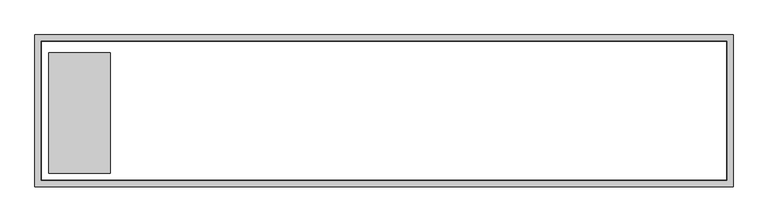
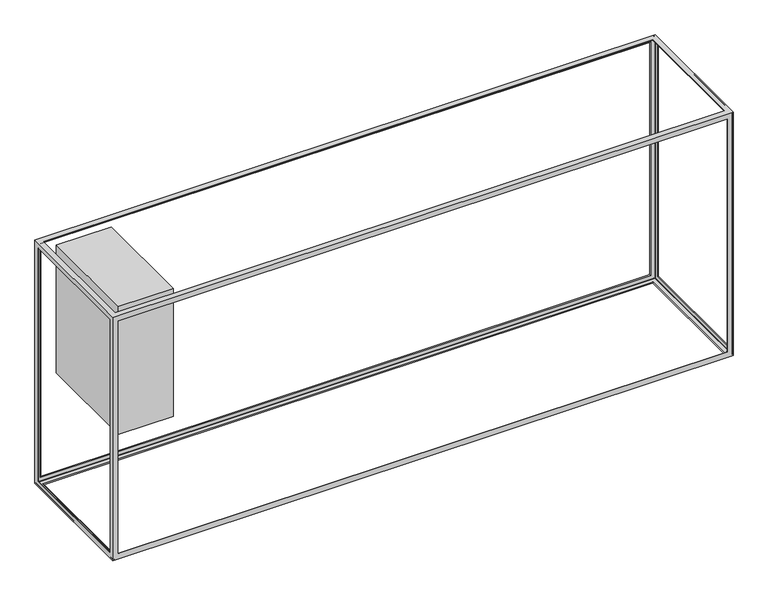
"""IFC4 building model written with IfcOpenShell, lengths in millimetres: beam geometry, Plumbing Bulkhead : EX. BULKHEAD 2."""

from ifc_helpers import new_model, si_unit, frame, origin, place, context, project, spatial, polyline, ellipse_curve, outline, extrude, source, transform, mapped, element, save
from ifc_brep_helpers import plane_surface, cylinder_surface, revolved_surface, advanced_brep


def beam_97812c56(model_context):
    return source(origin(), model_context, "Body", "SolidModel", [
        extrude(outline(polyline([(379.0365927, 673.1), (379.0365927, 66.5145898), (70.4236299, 66.5145898), (70.4236299, 673.1), (379.0365927, 673.1)])), frame((0.0, 0.0, 688.452765), z_axis=(0.0, 0.0, 1.0), x_axis=(1.0, 0.0, 0.0)), (0.0, 0.0, 1.0), 765.697235),
        advanced_brep(
        [(0.0, 0.0, 1454.15), (0.0, 762.0, 1454.15), (0.0, 762.0, 0.0), (0.0, 0.0, 0.0), (0.0, 31.75, 1422.4), (0.0, 31.75, 31.75), (0.0, 730.25, 31.75), (0.0, 730.25, 1422.4), (3505.2, 762.0, 1454.15), (3505.2, 762.0, 0.0), (3473.45, 762.0, 31.75), (3473.45, 762.0, 1422.4), (31.75, 762.0, 1422.4), (31.75, 762.0, 31.75), (3505.2, 0.0, 0.0), (3473.45, 730.25, 0.0), (31.75, 730.25, 0.0), (31.75, 31.75, 0.0), (3473.45, 31.75, 0.0), (3505.2, 0.0, 1454.15), (3473.45, 0.0, 1422.4), (3473.45, 0.0, 31.75), (31.75, 0.0, 31.75), (31.75, 0.0, 1422.4), (3.175, 28.575, 1425.575), (3.175, 28.575, 28.575), (3.175, 733.425, 28.575), (3.175, 733.425, 1425.575), (3505.2, 730.25, 31.75), (3502.025, 733.425, 28.575), (3502.025, 28.575, 28.575), (3505.2, 31.75, 31.75), (3505.2, 31.75, 1422.4), (3505.2, 730.25, 1422.4), (3502.025, 28.575, 1425.575), (3502.025, 733.425, 1425.575), (3476.625, 733.425, 3.175), (28.575, 733.425, 3.175), (28.575, 28.575, 3.175), (3476.625, 28.575, 3.175), (3500.4375, 4.7625, 3.175), (3500.4375, 757.2375, 3.175), (4.7625, 757.2375, 3.175), (4.7625, 4.7625, 3.175), (3501.560032, 758.360032, 3.639968), (3501.560032, 3.639968, 3.639968), (3502.025, 4.7625, 4.7625), (3502.025, 757.2375, 4.7625), (3500.4375, 758.825, 4.7625), (4.7625, 758.825, 4.7625), (3.639968, 758.360032, 3.639968), (3.175, 757.2375, 4.7625), (3.175, 4.7625, 4.7625), (3.639968, 3.639968, 3.639968), (4.7625, 3.175, 4.7625), (3500.4375, 3.175, 4.7625), (3500.4375, 758.825, 1449.3875), (4.7625, 758.825, 1449.3875), (3476.625, 758.825, 1425.575), (3476.625, 758.825, 28.575), (28.575, 758.825, 28.575), (28.575, 758.825, 1425.575), (3.639968, 758.360032, 1450.510032), (3.175, 757.2375, 1449.3875), (3502.025, 757.2375, 1449.3875), (3501.560032, 758.360032, 1450.510032), (3502.025, 4.7625, 1449.3875), (3500.4375, 3.175, 1449.3875), (3501.560032, 3.639968, 1450.510032), (3.175, 4.7625, 1449.3875), (4.7625, 3.175, 1449.3875), (3.639968, 3.639968, 1450.510032), (3476.625, 3.175, 1425.575), (3476.625, 3.175, 28.575), (28.575, 3.175, 28.575), (28.575, 3.175, 1425.575), (31.75, 31.75, 1454.15), (31.75, 730.25, 1454.15), (3473.45, 730.25, 1454.15), (3473.45, 31.75, 1454.15), (28.575, 733.425, 1450.975), (3476.625, 733.425, 1450.975), (4.7625, 4.7625, 1450.975), (4.7625, 757.2375, 1450.975), (3500.4375, 757.2375, 1450.975), (3500.4375, 4.7625, 1450.975), (28.575, 28.575, 1450.975), (3476.625, 28.575, 1450.975)],
        [
            (0, 1),
            (1, 2),
            (2, 3),
            (3, 0),
            (4, 5),
            (5, 6),
            (6, 7),
            (7, 4),
            (8, 9),
            (9, 2),
            (1, 8),
            (10, 11),
            (11, 12),
            (12, 13),
            (13, 10),
            (9, 14),
            (14, 3),
            (15, 16),
            (16, 17),
            (17, 18),
            (18, 15),
            (14, 19),
            (19, 0),
            (20, 21),
            (21, 22),
            (22, 23),
            (23, 20),
            (4, 24, ellipse_curve(frame((0.0, 28.575, 1425.575), z_axis=(0.0, -0.7071067811865464, -0.7071067811865487), x_axis=(0.0, 0.7071067811865487, -0.7071067811865464)), 4.4901281, 3.175)),
            (24, 25),
            (25, 5, ellipse_curve(frame((0.0, 28.575, 28.575), z_axis=(0.0, -0.7071067811865499, 0.7071067811865451), x_axis=(0.0, -0.7071067811865451, -0.7071067811865498)), 4.4901281, 3.175)),
            (25, 26),
            (26, 6, ellipse_curve(frame((0.0, 733.425, 28.575), z_axis=(0.0, -0.707106781186545, -0.70710678118655), x_axis=(0.0, -0.7071067811865501, 0.7071067811865449)), 4.4901281, 3.175)),
            (27, 7, ellipse_curve(frame((0.0, 733.425, 1425.575), z_axis=(0.0, 0.7071067811865487, -0.7071067811865464), x_axis=(0.0, -0.7071067811865465, -0.7071067811865487)), 4.4901281, 3.175)),
            (26, 27),
            (28, 29, ellipse_curve(frame((3505.2, 733.425, 28.575), z_axis=(0.0, -0.7071067811865429, -0.7071067811865522), x_axis=(0.0, -0.7071067811865521, 0.707106781186543)), 4.4901281, 3.175)),
            (29, 30),
            (30, 31, ellipse_curve(frame((3505.2, 28.575, 28.575), z_axis=(0.0, 0.7071067811865499, -0.7071067811865451), x_axis=(0.0, -0.7071067811865451, -0.70710678118655)), 4.4901281, 3.175)),
            (31, 28),
            (8, 19),
            (31, 32),
            (32, 33),
            (33, 28),
            (30, 34),
            (34, 32, ellipse_curve(frame((3505.2, 28.575, 1425.575), z_axis=(0.0, -0.7071067811865464, -0.7071067811865487), x_axis=(0.0, 0.7071067811865487, -0.7071067811865464)), 4.4901281, 3.175)),
            (33, 35, ellipse_curve(frame((3505.2, 733.425, 1425.575), z_axis=(0.0, 0.707106781186551, -0.7071067811865441), x_axis=(0.0, -0.7071067811865441, -0.7071067811865509)), 4.4901281, 3.175)),
            (35, 29),
            (15, 36, ellipse_curve(frame((3476.625, 733.425, 0.0), z_axis=(-0.7071067811865475, 0.7071067811865475, 0.0), x_axis=(-0.7071067811865476, -0.7071067811865474, 0.0)), 4.4901281, 3.175)),
            (36, 37),
            (37, 16, ellipse_curve(frame((28.575, 733.425, 0.0), z_axis=(0.7071067811865454, 0.7071067811865498, 0.0), x_axis=(-0.7071067811865497, 0.7071067811865454, 0.0)), 4.4901281, 3.175)),
            (37, 38),
            (38, 17, ellipse_curve(frame((28.575, 28.575, 0.0), z_axis=(-0.7071067811865498, 0.7071067811865452, 0.0), x_axis=(-0.7071067811865451, -0.7071067811865498, 0.0)), 4.4901281, 3.175)),
            (39, 18, ellipse_curve(frame((3476.625, 28.575, 0.0), z_axis=(-0.7071067811865475, -0.7071067811865475, 0.0), x_axis=(-0.7071067811865476, 0.7071067811865474, 0.0)), 4.4901281, 3.175)),
            (38, 39),
            (39, 36),
            (40, 41),
            (41, 42),
            (42, 43),
            (43, 40),
            (44, 41, ellipse_curve(frame((3500.4375, 757.2375, 4.7625), z_axis=(-0.7071067811865475, 0.7071067811865475, 0.0), x_axis=(0.7071067811865474, 0.7071067811865476, 0.0)), 2.245064, 1.5875)),
            (40, 45, ellipse_curve(frame((3500.4375, 4.7625, 4.7625), z_axis=(-0.7071067811865475, -0.7071067811865475, 0.0), x_axis=(-0.7071067811865474, 0.7071067811865476, 0.0)), 2.245064, 1.5875)),
            (45, 46, ellipse_curve(frame((3500.4375, 4.7625, 4.7625), z_axis=(0.0, -0.7071067811865499, 0.7071067811865451), x_axis=(0.0, 0.7071067811865451, 0.70710678118655)), 2.245064, 1.5875)),
            (46, 47),
            (47, 44, ellipse_curve(frame((3500.4375, 757.2375, 4.7625), z_axis=(0.0, 0.7071067811865429, 0.7071067811865522), x_axis=(0.0, 0.7071067811865521, -0.707106781186543)), 2.245064, 1.5875)),
            (48, 49),
            (49, 50, ellipse_curve(frame((4.7625, 757.2375, 4.7625), z_axis=(-0.7071067811865439, 0.0, 0.7071067811865511), x_axis=(0.7071067811865511, 0.0, 0.7071067811865438)), 2.245064, 1.5875)),
            (50, 42, ellipse_curve(frame((4.7625, 757.2375, 4.7625), z_axis=(-0.7071067811865454, -0.7071067811865498, 0.0), x_axis=(0.7071067811865497, -0.7071067811865454, 0.0)), 2.245064, 1.5875)),
            (44, 48, ellipse_curve(frame((3500.4375, 757.2375, 4.7625), z_axis=(0.7071067811865475, 0.0, 0.7071067811865476), x_axis=(0.7071067811865475, 0.0, -0.7071067811865475)), 2.245064, 1.5875)),
            (51, 52),
            (52, 53, ellipse_curve(frame((4.7625, 4.7625, 4.7625), z_axis=(0.0, -0.7071067811865499, 0.7071067811865451), x_axis=(0.0, 0.7071067811865451, 0.70710678118655)), 2.245064, 1.5875)),
            (53, 43, ellipse_curve(frame((4.7625, 4.7625, 4.7625), z_axis=(0.7071067811865498, -0.7071067811865452, 0.0), x_axis=(0.7071067811865451, 0.7071067811865498, 0.0)), 2.245064, 1.5875)),
            (50, 51, ellipse_curve(frame((4.7625, 757.2375, 4.7625), z_axis=(0.0, 0.707106781186545, 0.70710678118655), x_axis=(0.0, 0.7071067811865501, -0.7071067811865449)), 2.245064, 1.5875)),
            (53, 54, ellipse_curve(frame((4.7625, 4.7625, 4.7625), z_axis=(-0.7071067811865439, 0.0, 0.7071067811865511), x_axis=(0.7071067811865511, 0.0, 0.7071067811865438)), 2.245064, 1.5875)),
            (54, 55),
            (55, 45, ellipse_curve(frame((3500.4375, 4.7625, 4.7625), z_axis=(0.7071067811865475, 0.0, 0.7071067811865476), x_axis=(0.7071067811865475, 0.0, -0.7071067811865475)), 2.245064, 1.5875)),
            (48, 56),
            (56, 57),
            (57, 49),
            (58, 59),
            (59, 60),
            (60, 61),
            (61, 58),
            (57, 62, ellipse_curve(frame((4.7625, 757.2375, 1449.3875), z_axis=(0.7071067811865511, 0.0, 0.7071067811865439), x_axis=(-0.7071067811865438, 0.0, 0.7071067811865511)), 2.245064, 1.5875)),
            (62, 63, ellipse_curve(frame((4.7625, 757.2375, 1449.3875), z_axis=(0.0, -0.7071067811865487, 0.7071067811865464), x_axis=(0.0, 0.7071067811865465, 0.7071067811865487)), 2.245064, 1.5875)),
            (63, 51),
            (47, 64),
            (64, 65, ellipse_curve(frame((3500.4375, 757.2375, 1449.3875), z_axis=(0.0, -0.707106781186551, 0.7071067811865441), x_axis=(0.0, 0.7071067811865441, 0.7071067811865509)), 2.245064, 1.5875)),
            (65, 56, ellipse_curve(frame((3500.4375, 757.2375, 1449.3875), z_axis=(-0.7071067811865475, 0.0, 0.7071067811865475), x_axis=(0.7071067811865474, 0.0, 0.7071067811865476)), 2.245064, 1.5875)),
            (10, 59, ellipse_curve(frame((3476.625, 762.0, 28.575), z_axis=(0.7071067811865475, 0.0, 0.7071067811865476), x_axis=(0.7071067811865476, 0.0, -0.7071067811865475)), 4.4901281, 3.175)),
            (58, 11, ellipse_curve(frame((3476.625, 762.0, 1425.575), z_axis=(0.7071067811865475, 0.0, -0.7071067811865475), x_axis=(-0.7071067811865474, 0.0, -0.7071067811865476)), 4.4901281, 3.175)),
            (13, 60, ellipse_curve(frame((28.575, 762.0, 28.575), z_axis=(0.7071067811865439, 0.0, -0.7071067811865511), x_axis=(-0.7071067811865511, 0.0, -0.7071067811865438)), 4.4901281, 3.175)),
            (12, 61, ellipse_curve(frame((28.575, 762.0, 1425.575), z_axis=(-0.7071067811865511, 0.0, -0.7071067811865439), x_axis=(0.7071067811865438, 0.0, -0.7071067811865511)), 4.4901281, 3.175)),
            (46, 66),
            (66, 64),
            (35, 34),
            (55, 67),
            (67, 68, ellipse_curve(frame((3500.4375, 4.7625, 1449.3875), z_axis=(-0.7071067811865475, 0.0, 0.7071067811865475), x_axis=(0.7071067811865474, 0.0, 0.7071067811865476)), 2.245064, 1.5875)),
            (68, 66, ellipse_curve(frame((3500.4375, 4.7625, 1449.3875), z_axis=(0.0, 0.7071067811865464, 0.7071067811865487), x_axis=(0.0, -0.7071067811865487, 0.7071067811865464)), 2.245064, 1.5875)),
            (63, 69),
            (69, 52),
            (24, 27),
            (70, 54),
            (69, 71, ellipse_curve(frame((4.7625, 4.7625, 1449.3875), z_axis=(0.0, 0.7071067811865464, 0.7071067811865487), x_axis=(0.0, -0.7071067811865487, 0.7071067811865464)), 2.245064, 1.5875)),
            (71, 70, ellipse_curve(frame((4.7625, 4.7625, 1449.3875), z_axis=(0.7071067811865511, 0.0, 0.7071067811865439), x_axis=(-0.7071067811865438, 0.0, 0.7071067811865511)), 2.245064, 1.5875)),
            (72, 73),
            (73, 21, ellipse_curve(frame((3476.625, 0.0, 28.575), z_axis=(0.7071067811865475, 0.0, 0.7071067811865476), x_axis=(0.7071067811865476, 0.0, -0.7071067811865475)), 4.4901281, 3.175)),
            (20, 72, ellipse_curve(frame((3476.625, 0.0, 1425.575), z_axis=(0.7071067811865475, 0.0, -0.7071067811865475), x_axis=(-0.7071067811865474, 0.0, -0.7071067811865476)), 4.4901281, 3.175)),
            (73, 74),
            (74, 22, ellipse_curve(frame((28.575, 0.0, 28.575), z_axis=(0.7071067811865439, 0.0, -0.7071067811865511), x_axis=(-0.7071067811865511, 0.0, -0.7071067811865438)), 4.4901281, 3.175)),
            (74, 75),
            (75, 23, ellipse_curve(frame((28.575, 0.0, 1425.575), z_axis=(-0.7071067811865511, 0.0, -0.7071067811865439), x_axis=(0.7071067811865438, 0.0, -0.7071067811865511)), 4.4901281, 3.175)),
            (70, 67),
            (72, 75),
            (76, 77),
            (77, 78),
            (78, 79),
            (79, 76),
            (77, 80, ellipse_curve(frame((28.575, 733.425, 1454.15), z_axis=(0.707106781186548, 0.7071067811865469, 0.0), x_axis=(-0.707106781186547, 0.7071067811865478, 0.0)), 4.4901281, 3.175)),
            (80, 81),
            (81, 78, ellipse_curve(frame((3476.625, 733.425, 1454.15), z_axis=(-0.7071067811865469, 0.707106781186548, 0.0), x_axis=(-0.7071067811865481, -0.7071067811865468, 0.0)), 4.4901281, 3.175)),
            (82, 83),
            (83, 84),
            (84, 85),
            (85, 82),
            (80, 86),
            (86, 87),
            (87, 81),
            (65, 84, ellipse_curve(frame((3500.4375, 757.2375, 1449.3875), z_axis=(0.7071067811865469, -0.707106781186548, 0.0), x_axis=(0.7071067811865481, 0.7071067811865468, 0.0)), 2.245064, 1.5875)),
            (83, 62, ellipse_curve(frame((4.7625, 757.2375, 1449.3875), z_axis=(-0.707106781186548, -0.7071067811865469, 0.0), x_axis=(0.707106781186547, -0.7071067811865478, 0.0)), 2.245064, 1.5875)),
            (86, 76, ellipse_curve(frame((28.575, 28.575, 1454.15), z_axis=(0.7071067811865469, -0.707106781186548, 0.0), x_axis=(-0.7071067811865481, -0.7071067811865468, 0.0)), 4.4901281, 3.175)),
            (79, 87, ellipse_curve(frame((3476.625, 28.575, 1454.15), z_axis=(-0.707106781186548, -0.7071067811865469, 0.0), x_axis=(-0.707106781186547, 0.7071067811865478, 0.0)), 4.4901281, 3.175)),
            (71, 82, ellipse_curve(frame((4.7625, 4.7625, 1449.3875), z_axis=(-0.7071067811865469, 0.707106781186548, 0.0), x_axis=(0.7071067811865481, 0.7071067811865468, 0.0)), 2.245064, 1.5875)),
            (85, 68, ellipse_curve(frame((3500.4375, 4.7625, 1449.3875), z_axis=(0.707106781186548, 0.7071067811865469, 0.0), x_axis=(0.707106781186547, -0.7071067811865478, 0.0)), 2.245064, 1.5875)),
        ],
        [
            plane_surface(frame((0.0, 762.0, 0.0), z_axis=(-1.0, 0.0, 0.0), x_axis=(0.0, 0.0, 1.0))),
            plane_surface(frame((0.0, 762.0, 31.75), z_axis=(0.0, 1.0, 0.0), x_axis=(1.0, 0.0, 0.0))),
            plane_surface(frame((0.0, 762.0, 0.0), z_axis=(0.0, 0.0, -1.0), x_axis=(1.0, 0.0, 0.0))),
            plane_surface(frame((3505.2, 0.0, 0.0), z_axis=(0.0, -1.0, 0.0), x_axis=(0.0, 0.0, 1.0))),
            cylinder_surface(frame((0.0, 28.575, 0.0), z_axis=(0.0, 0.0, -1.0), x_axis=(0.0, 1.0, 0.0)), 3.175),
            cylinder_surface(frame((0.0, 0.0, 28.575), z_axis=(0.0, -1.0, 0.0), x_axis=(1.0, 0.0, 0.0)), 3.175),
            cylinder_surface(frame((0.0, 733.425, 0.0), z_axis=(0.0, 0.0, -1.0), x_axis=(0.0, -1.0, 0.0)), 3.175),
            cylinder_surface(frame((3505.2, 0.0, 28.575), z_axis=(0.0, -1.0, 0.0), x_axis=(-1.0, 0.0, 0.0)), 3.175),
            plane_surface(frame((3505.2, 762.0, 0.0), z_axis=(1.0, 0.0, 0.0), x_axis=(0.0, 0.0, 1.0))),
            cylinder_surface(frame((3505.2, 28.575, 0.0), z_axis=(0.0, 0.0, -1.0), x_axis=(0.0, 1.0, 0.0)), 3.175),
            cylinder_surface(frame((3505.2, 733.425, 0.0), z_axis=(0.0, 0.0, -1.0), x_axis=(0.0, -1.0, 0.0)), 3.175),
            cylinder_surface(frame((0.0, 733.425, 0.0), z_axis=(-1.0, 0.0, 0.0), x_axis=(0.0, -1.0, 0.0)), 3.175),
            cylinder_surface(frame((28.575, 0.0, 0.0), z_axis=(0.0, -1.0, 0.0), x_axis=(1.0, 0.0, 0.0)), 3.175),
            cylinder_surface(frame((0.0, 28.575, 0.0), z_axis=(-1.0, 0.0, 0.0), x_axis=(0.0, 1.0, 0.0)), 3.175),
            cylinder_surface(frame((3476.625, 0.0, 0.0), z_axis=(0.0, -1.0, 0.0), x_axis=(-1.0, 0.0, 0.0)), 3.175),
            plane_surface(frame((0.0, 733.425, 3.175), z_axis=(0.0, 0.0, 1.0), x_axis=(1.0, 0.0, 0.0))),
            revolved_surface(polyline([(3498.85, 758.8249999785978, 4.7625), (3498.85, 3.1750000214022047, 4.7625)]), (3500.4375, 0.0, 4.7625), (0.0, 1.0, 0.0)),
            revolved_surface(polyline([(3502.024999978598, 755.65, 4.7625), (3.175000021402197, 755.65, 4.7625)]), (0.0, 757.2375, 4.7625), (1.0, 0.0, 0.0)),
            revolved_surface(polyline([(6.35, 758.8249999785977, 4.7625), (6.35, 3.1750000214022, 4.7625)]), (4.7625, 0.0, 4.7625), (0.0, 1.0, 0.0)),
            revolved_surface(polyline([(3502.024999978598, 6.35, 4.7625), (3.175000021402197, 6.35, 4.7625)]), (0.0, 4.7625, 4.7625), (1.0, 0.0, 0.0)),
            plane_surface(frame((0.0, 758.825, 4.7625), z_axis=(0.0, -1.0, 0.0), x_axis=(1.0, 0.0, 0.0))),
            revolved_surface(polyline([(4.7625, 755.65, 1450.974999978598), (4.7625, 755.65, 3.1750000214022105)]), (4.7625, 757.2375, 0.0), (0.0, 0.0, 1.0)),
            revolved_surface(polyline([(3500.4375, 755.65, 1450.974999978598), (3500.4375, 755.65, 3.175000021402205)]), (3500.4375, 757.2375, 0.0), (0.0, 0.0, 1.0)),
            cylinder_surface(frame((3476.625, 762.0, 0.0), z_axis=(0.0, 0.0, -1.0), x_axis=(0.0, -1.0, 0.0)), 3.175),
            cylinder_surface(frame((0.0, 762.0, 28.575), z_axis=(-1.0, 0.0, 0.0), x_axis=(0.0, -1.0, 0.0)), 3.175),
            cylinder_surface(frame((28.575, 762.0, 0.0), z_axis=(0.0, 0.0, -1.0), x_axis=(0.0, -1.0, 0.0)), 3.175),
            plane_surface(frame((3502.025, 733.425, 0.0), z_axis=(-1.0, 0.0, 0.0), x_axis=(0.0, 0.0, 1.0))),
            revolved_surface(polyline([(3500.4375, 6.35, 1450.974999978598), (3500.4375, 6.35, 3.1750000214021994)]), (3500.4375, 4.7625, 0.0), (0.0, 0.0, 1.0)),
            plane_surface(frame((3.175, 757.2375, 0.0), z_axis=(1.0, 0.0, 0.0), x_axis=(0.0, 0.0, 1.0))),
            revolved_surface(polyline([(4.7625, 6.35, 1450.974999978598), (4.7625, 6.35, 3.1750000214021994)]), (4.7625, 4.7625, 0.0), (0.0, 0.0, 1.0)),
            cylinder_surface(frame((3476.625, 0.0, 0.0), z_axis=(0.0, 0.0, -1.0), x_axis=(0.0, 1.0, 0.0)), 3.175),
            cylinder_surface(frame((0.0, 0.0, 28.575), z_axis=(-1.0, 0.0, 0.0), x_axis=(0.0, 1.0, 0.0)), 3.175),
            cylinder_surface(frame((28.575, 0.0, 0.0), z_axis=(0.0, 0.0, -1.0), x_axis=(0.0, 1.0, 0.0)), 3.175),
            plane_surface(frame((0.0, 3.175, 1449.3875), z_axis=(0.0, 1.0, 0.0), x_axis=(1.0, 0.0, 0.0))),
            plane_surface(frame((3505.2, 762.0, 1454.15), z_axis=(0.0, 0.0, 1.0), x_axis=(1.0, 0.0, 0.0))),
            cylinder_surface(frame((0.0, 733.425, 1454.15), z_axis=(-1.0, 0.0, 0.0), x_axis=(0.0, -1.0, 0.0)), 3.175),
            plane_surface(frame((0.0, 757.2375, 1450.975), z_axis=(0.0, 0.0, -1.0), x_axis=(1.0, 0.0, 0.0))),
            revolved_surface(polyline([(3502.024999978598, 755.65, 1449.3875), (3.175000021402206, 755.65, 1449.3875)]), (0.0, 757.2375, 1449.3875), (1.0, 0.0, 0.0)),
            cylinder_surface(frame((0.0, 762.0, 1425.575), z_axis=(-1.0, 0.0, 0.0), x_axis=(0.0, -1.0, 0.0)), 3.175),
            cylinder_surface(frame((0.0, 28.575, 1454.15), z_axis=(-1.0, 0.0, 0.0), x_axis=(0.0, 1.0, 0.0)), 3.175),
            revolved_surface(polyline([(3502.024999978598, 6.35, 1449.3875), (3.1750000214022034, 6.35, 1449.3875)]), (0.0, 4.7625, 1449.3875), (1.0, 0.0, 0.0)),
            cylinder_surface(frame((0.0, 0.0, 1425.575), z_axis=(-1.0, 0.0, 0.0), x_axis=(0.0, 1.0, 0.0)), 3.175),
            cylinder_surface(frame((28.575, 0.0, 1454.15), z_axis=(0.0, -1.0, 0.0), x_axis=(1.0, 0.0, 0.0)), 3.175),
            revolved_surface(polyline([(6.35, 758.8249999785977, 1449.3875), (6.35, 3.1750000214022025, 1449.3875)]), (4.7625, 0.0, 1449.3875), (0.0, 1.0, 0.0)),
            cylinder_surface(frame((0.0, 0.0, 1425.575), z_axis=(0.0, -1.0, 0.0), x_axis=(1.0, 0.0, 0.0)), 3.175),
            cylinder_surface(frame((3476.625, 0.0, 1454.15), z_axis=(0.0, -1.0, 0.0), x_axis=(-1.0, 0.0, 0.0)), 3.175),
            revolved_surface(polyline([(3498.85, 758.8249999785977, 1449.3875), (3498.85, 3.1750000214022025, 1449.3875)]), (3500.4375, 0.0, 1449.3875), (0.0, 1.0, 0.0)),
            cylinder_surface(frame((3505.2, 0.0, 1425.575), z_axis=(0.0, -1.0, 0.0), x_axis=(-1.0, 0.0, 0.0)), 3.175),
        ],
        [
            (0, [[1, 2, 3, 4], [5, 6, 7, 8]]),
            (1, [[9, 10, -2, 11], [12, 13, 14, 15]]),
            (2, [[-3, -10, 16, 17], [18, 19, 20, 21]]),
            (3, [[-17, 22, 23, -4], [24, 25, 26, 27]]),
            (4, [[28, 29, 30, -5]]),
            (5, [[31, 32, -6, -30]]),
            (6, [[33, -7, -32, 34]]),
            (7, [[35, 36, 37, 38]]),
            (8, [[-16, -9, 39, -22], [-38, 40, 41, 42]]),
            (9, [[-37, 43, 44, -40]]),
            (10, [[-35, -42, 45, 46]]),
            (11, [[47, 48, 49, -18]]),
            (12, [[-19, -49, 50, 51]]),
            (13, [[52, -20, -51, 53]]),
            (14, [[-47, -21, -52, 54]]),
            (15, [[55, 56, 57, 58], [-54, -53, -50, -48]]),
            (16, [[59, -55, 60, 61, 62, 63]]),
            (17, [[64, 65, 66, -56, -59, 67]]),
            (18, [[68, 69, 70, -57, -66, 71]]),
            (19, [[-60, -58, -70, 72, 73, 74]]),
            (20, [[75, 76, 77, -64], [78, 79, 80, 81]]),
            (21, [[-77, 82, 83, 84, -71, -65]]),
            (22, [[-75, -67, -63, 85, 86, 87]]),
            (23, [[88, -78, 89, -12]]),
            (24, [[-88, -15, 90, -79]]),
            (25, [[-80, -90, -14, 91]]),
            (26, [[-62, 92, 93, -85], [-36, -46, 94, -43]]),
            (27, [[-61, -74, 95, 96, 97, -92]]),
            (28, [[98, 99, -68, -84], [100, -34, -31, -29]]),
            (29, [[101, -72, -69, -99, 102, 103]]),
            (30, [[104, 105, -24, 106]]),
            (31, [[-105, 107, 108, -25]]),
            (32, [[109, 110, -26, -108]]),
            (33, [[-95, -73, -101, 111], [-104, 112, -109, -107]]),
            (34, [[-1, -23, -39, -11], [113, 114, 115, 116]]),
            (35, [[117, 118, 119, -114]]),
            (36, [[120, 121, 122, 123], [124, 125, 126, -118]]),
            (37, [[-76, -87, 127, -121, 128, -82]]),
            (38, [[-89, -81, -91, -13]]),
            (39, [[129, -116, 130, -125]]),
            (40, [[-111, -103, 131, -123, 132, -96]]),
            (41, [[-106, -27, -110, -112]]),
            (42, [[-113, -129, -124, -117]]),
            (43, [[-128, -120, -131, -102, -98, -83]]),
            (44, [[-8, -33, -100, -28]]),
            (45, [[-126, -130, -115, -119]]),
            (46, [[-86, -93, -97, -132, -122, -127]]),
            (47, [[-41, -44, -94, -45]]),
        ],
    ),
    ])


if __name__ == "__main__":
    model = new_model("IFC4")
    model_context = context("Model", 3, world=origin())
    ifc_project = project(units=[si_unit("LENGTHUNIT", "METRE", prefix="MILLI")], contexts=[model_context])
    site = spatial("IfcSite", under=ifc_project)
    building = spatial("IfcBuilding", under=site)
    placement = place(None, origin())
    beam_shape = beam_97812c56(model_context)
    element("IfcBeam", 1, ObjectType="Plumbing Bulkhead : EX. BULKHEAD 2", at=placement, inside=building, context=model_context, shape_type="MappedRepresentation", body=[
        mapped(beam_shape, transform((0.0, 0.0, 0.0), x_axis=(1.0, 0.0, 0.0), y_axis=(0.0, 1.0, 0.0), z_axis=(0.0, 0.0, 1.0))),
    ])
    save(model, "model.ifc")

# Revit data of these elements
# Type "Plumbing Bulkhead : EX. BULKHEAD 2"
#   Length = 11' - 6"
#   Height = 4' - 9 1/4"
#   Depth = 2' - 6"
#   Structural Material = USE EXISTING BULKHEADS IN STORAGE (MODIFY AS NECESSARY)
#   EP MATERIAL = ELECTRICAL PANEL
# Element 1 (IfcBeam, "Plumbing Bulkhead : EX. BULKHEAD 2")
#   Materials on its faces: "USE EXISTING BULKHEADS IN STORAGE (MODIFY AS NECESSARY)", "ELECTRICAL PANEL"
# Materials
#   "USE EXISTING BULKHEADS IN STORAGE (MODIFY AS NECESSARY)": class "Generic", colour RGB 120 120 120, transparency 0, Cost = 0
#   "ELECTRICAL PANEL": class "Generic", colour RGB 255 255 255, transparency 0, Cost = 0
